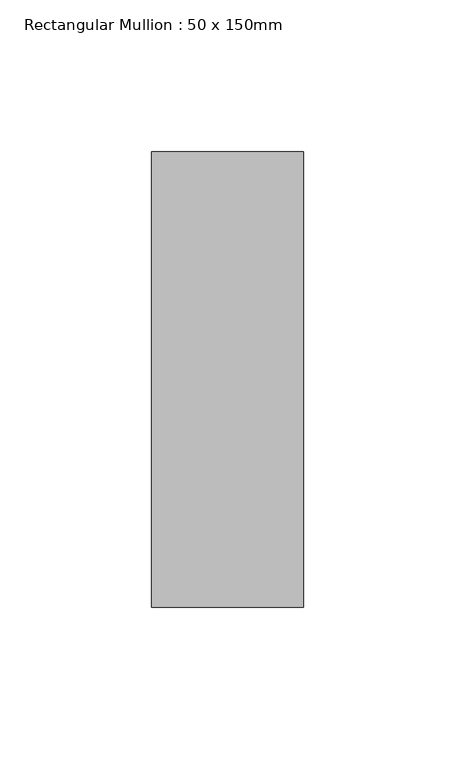
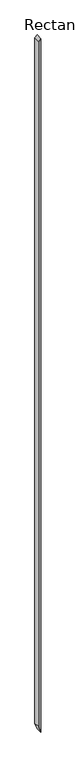
"""IFC4 building model written with IfcOpenShell, lengths in millimetres: member geometry, Rectangular Mullion : 50 x 150mm."""

from ifc_helpers import new_model, si_unit, frame, origin, place, context, project, spatial, polyline, outline, extrude, source, transform, mapped, element, save


def rectangular_mullion_50_x_150mm_d02c79f9(model_context):
    return source(origin(), model_context, "Body", "SweptSolid", [
        extrude(outline(polyline([(0.0, 0.0), (-53.1084457, -50.0), (-16559.0646109, -50.0), (-16709.3575071, 0.0), (0.0, 0.0)])), frame((0.0, -75.0, 0.0), z_axis=(0.0, 1.0, 0.0), x_axis=(0.0, 0.0, 1.0)), (0.0, 0.0, 1.0), 150.0),
    ])


if __name__ == "__main__":
    model = new_model("IFC4")
    model_context = context("Model", 3, world=origin())
    ifc_project = project(units=[si_unit("LENGTHUNIT", "METRE", prefix="MILLI")], contexts=[model_context])
    site = spatial("IfcSite", under=ifc_project)
    building = spatial("IfcBuilding", under=site)
    placement = place(None, origin())
    rectangular_mullion_50_x_150mm_shape = rectangular_mullion_50_x_150mm_d02c79f9(model_context)
    element("IfcMember", 1, ObjectType="Rectangular Mullion : 50 x 150mm", at=placement, inside=building, context=model_context, shape_type="MappedRepresentation", body=[
        mapped(rectangular_mullion_50_x_150mm_shape, transform((0.0, 0.0, 0.0), x_axis=(1.0, 0.0, 0.0), y_axis=(0.0, 1.0, 0.0), z_axis=(0.0, 0.0, 1.0))),
    ])
    save(model, "model.ifc")

# Revit data of these elements
# Type "Rectangular Mullion : 50 x 150mm"
#   built-in parameter 1007304 = 0.492126 (stored number, unit not read)
#   built-in parameter 1007301 = 0.082021 (stored number, unit not read)
#   built-in parameter 1007300 = 0.082021 (stored number, unit not read)
# Element 1 (IfcMember, "Rectangular Mullion : 50 x 150mm")
#   Materials on its faces: "Metal - Aluminium"
# Materials
#   "Metal - Aluminium": class "Metal", colour RGB 247 247 247, transparency 0
